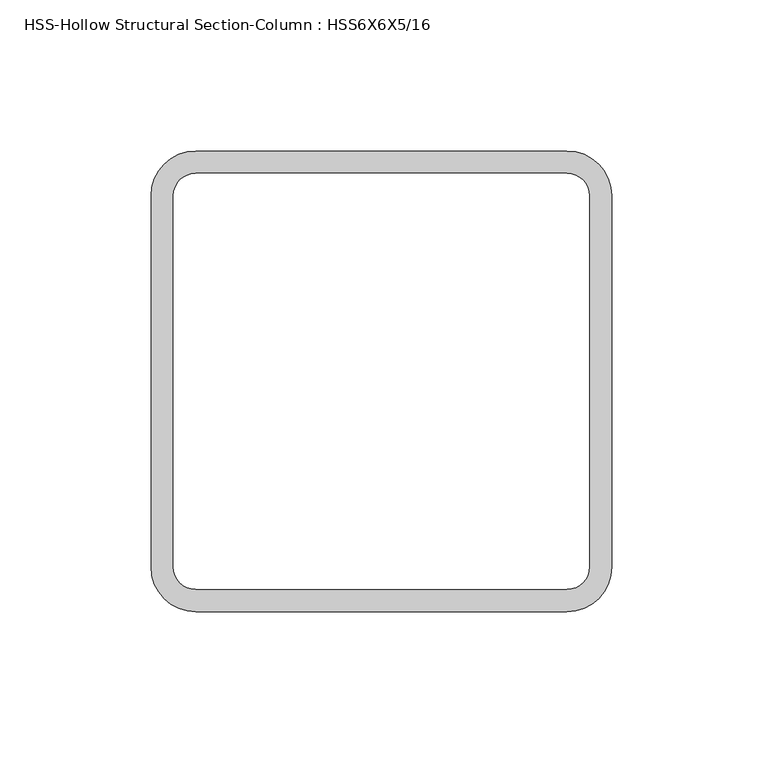
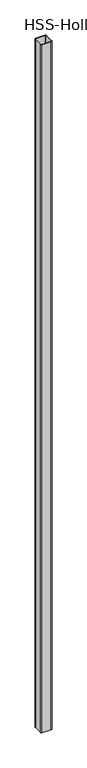
"""IFC4 building model written with IfcOpenShell, lengths in millimetres: column geometry, HSS-Hollow Structural Section-Column : HSS6X6X5/16."""

from ifc_helpers import new_model, si_unit, point, frame, frame_2d, origin, place, context, project, spatial, polyline, circle_curve, trimmed, segment, composite_curve, outline, extrude, source, transform, mapped, element, save


def hss_hollow_structural_section_column_hss6x6x5_16_20d757cc(model_context):
    return source(origin(), model_context, "Body", "SweptSolid", [
        extrude(outline(composite_curve([segment(trimmed(circle_curve(frame_2d((61.4172, 61.4172)), 14.7828), [point((61.4172, 76.2))], [point((76.2, 61.4172))], False, "CARTESIAN"), True, "CONTINUOUS"), segment(polyline([(76.2, 61.4172), (76.2, -61.4172)]), True, "CONTINUOUS"), segment(trimmed(circle_curve(frame_2d((61.4172, -61.4172)), 14.7828), [point((76.2, -61.4172))], [point((61.4172, -76.2))], False, "CARTESIAN"), True, "CONTINUOUS"), segment(polyline([(61.4172, -76.2), (-61.4172, -76.2)]), True, "CONTINUOUS"), segment(trimmed(circle_curve(frame_2d((-61.4172, -61.4172)), 14.7828), [point((-61.4172, -76.2))], [point((-76.2, -61.4172))], False, "CARTESIAN"), True, "CONTINUOUS"), segment(polyline([(-76.2, -61.4172), (-76.2, 61.4172)]), True, "CONTINUOUS"), segment(trimmed(circle_curve(frame_2d((-61.4172, 61.4172)), 14.7828), [point((-76.2, 61.4172))], [point((-61.4172, 76.2))], False, "CARTESIAN"), True, "CONTINUOUS"), segment(polyline([(-61.4172, 76.2), (61.4172, 76.2)]), True, "CONTINUOUS")], self_intersect=False), holes=[composite_curve([segment(polyline([(61.4172, 68.8086), (-61.4172, 68.8086)]), True, "CONTINUOUS"), segment(trimmed(circle_curve(frame_2d((-61.4172, 61.4172)), 7.3914), [point((-61.4172, 68.8086))], [point((-68.8086, 61.4172))], True, "CARTESIAN"), True, "CONTINUOUS"), segment(polyline([(-68.8086, 61.4172), (-68.8086, -61.4172)]), True, "CONTINUOUS"), segment(trimmed(circle_curve(frame_2d((-61.4172, -61.4172)), 7.3914), [point((-68.8086, -61.4172))], [point((-61.4172, -68.8086))], True, "CARTESIAN"), True, "CONTINUOUS"), segment(polyline([(-61.4172, -68.8086), (61.4172, -68.8086)]), True, "CONTINUOUS"), segment(trimmed(circle_curve(frame_2d((61.4172, -61.4172)), 7.3914), [point((61.4172, -68.8086))], [point((68.8086, -61.4172))], True, "CARTESIAN"), True, "CONTINUOUS"), segment(polyline([(68.8086, -61.4172), (68.8086, 61.4172)]), True, "CONTINUOUS"), segment(trimmed(circle_curve(frame_2d((61.4172, 61.4172)), 7.3914), [point((68.8086, 61.4172))], [point((61.4172, 68.8086))], True, "CARTESIAN"), True, "CONTINUOUS")], self_intersect=False)]), frame((0.0, 0.0, 17627.6), z_axis=(0.0, 0.0, 1.0), x_axis=(1.0, 0.0, 0.0)), (0.0, 0.0, 1.0), 9956.8),
    ])


if __name__ == "__main__":
    model = new_model("IFC4")
    model_context = context("Model", 3, world=origin())
    ifc_project = project(units=[si_unit("LENGTHUNIT", "METRE", prefix="MILLI")], contexts=[model_context])
    site = spatial("IfcSite", under=ifc_project)
    building = spatial("IfcBuilding", under=site)
    placement = place(None, origin())
    hss_hollow_structural_section_column_hss6x6x5_16_shape = hss_hollow_structural_section_column_hss6x6x5_16_20d757cc(model_context)
    element("IfcColumn", 1, ObjectType="HSS-Hollow Structural Section-Column : HSS6X6X5/16", at=placement, inside=building, context=model_context, shape_type="MappedRepresentation", body=[
        mapped(hss_hollow_structural_section_column_hss6x6x5_16_shape, transform((0.0, 0.0, 0.0), x_axis=(1.0, 0.0, 0.0), y_axis=(0.0, 1.0, 0.0), z_axis=(0.0, 0.0, 1.0))),
    ])
    save(model, "model.ifc")

# Revit data of these elements
# Type "HSS-Hollow Structural Section-Column : HSS6X6X5/16"
#   Assembly Code = "B10"
#   Shape = "Square"
#   W = 23.3
#   Ht = 0' - 6"
#   b = 0' - 6"
#   kr = 0' - 0.582"
#   t = 0' - 0.291"
#   A = 0.0446528 SF
#   Structural Material [instance default] = Steel ASTM A500, Grade B, Rectangular and Square
# Element 1 (IfcColumn, "HSS-Hollow Structural Section-Column : HSS6X6X5/16")
#   Materials on its faces: "Steel ASTM A500, Grade B, Rectangular and Square"
# Materials
#   "Steel ASTM A500, Grade B, Rectangular and Square": class "Metal", colour RGB 199 199 199, transparency 0, Description = "Carbon steel", Cost = 0
